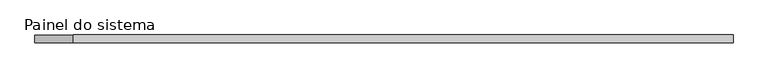
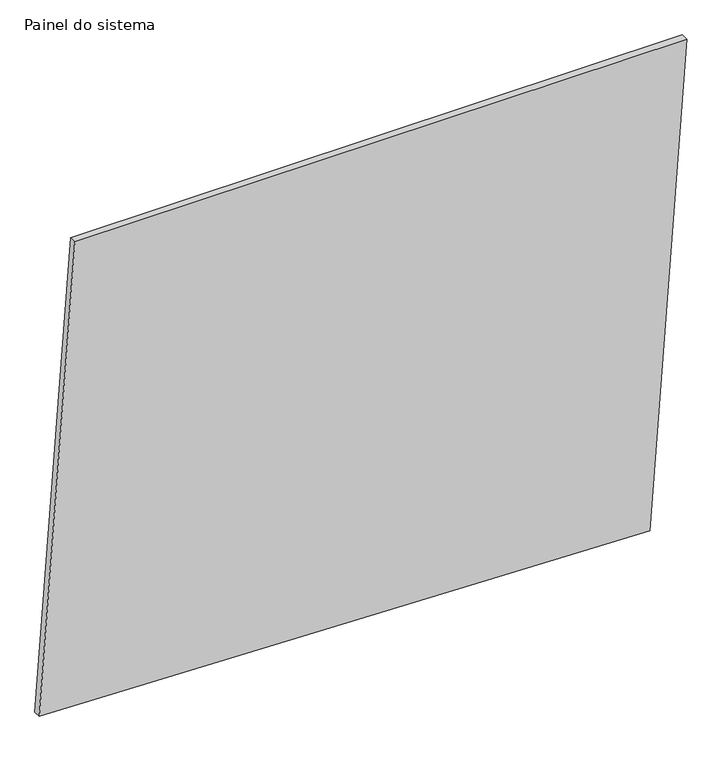
"""IFC4 building model written with IfcOpenShell, lengths in millimetres: plate geometry, Painel do sistema : Envidraçado."""

from ifc_helpers import new_model, si_unit, frame, origin, place, context, project, spatial, polyline, outline, extrude, source, transform, mapped, element, save


def painel_do_sistema_84858c02(model_context):
    return source(origin(), model_context, "Body", "SweptSolid", [
        extrude(outline(polyline([(59.4199302, -1093.7911549), (0.0, 969.1976394), (1710.7366656, 1093.7911549), (1710.7366656, -973.5252125), (59.4199302, -1093.7911549)])), frame((0.0, 24.5, 0.0), z_axis=(0.0, 1.0, 0.0), x_axis=(0.0, 0.0, 1.0)), (0.0, 0.0, 1.0), 25.0),
    ])


if __name__ == "__main__":
    model = new_model("IFC4")
    model_context = context("Model", 3, world=origin())
    ifc_project = project(units=[si_unit("LENGTHUNIT", "METRE", prefix="MILLI")], contexts=[model_context])
    site = spatial("IfcSite", under=ifc_project)
    building = spatial("IfcBuilding", under=site)
    placement = place(None, origin())
    painel_do_sistema_shape = painel_do_sistema_84858c02(model_context)
    element("IfcPlate", 1, ObjectType="Painel do sistema : Envidraçado", at=placement, inside=building, context=model_context, shape_type="MappedRepresentation", body=[
        mapped(painel_do_sistema_shape, transform((0.0, 0.0, 0.0), x_axis=(1.0, 0.0, 0.0), y_axis=(0.0, 1.0, 0.0), z_axis=(0.0, 0.0, 1.0))),
    ])
    save(model, "model.ifc")

# Revit data of these elements
# Type "Painel do sistema : Envidraçado"
#   Construction Type Id = "GSP4R"
#   Analytic Construction = "Vidraça única Pilkington 1/8 pol"
#   Visual Light Transmittance = 0.9
#   Solar Heat Gain Coefficient = 0.86
#   Heat Transfer Coefficient (U) = 6.7069 W/(m²·K)
# Element 1 (IfcPlate, "Painel do sistema : Envidraçado")
#   Materials on its faces: "Vidro"
# Materials
#   "Vidro": class "Vidro", colour RGB 0 128 192, transparency 0.9, Description = "Vidro de sílica", Cost = 0
